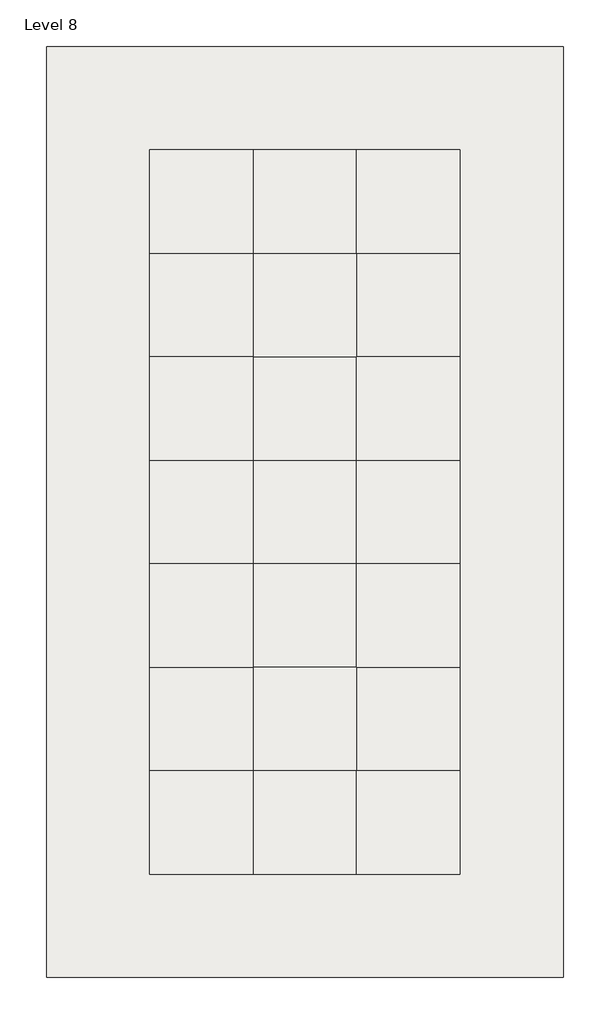
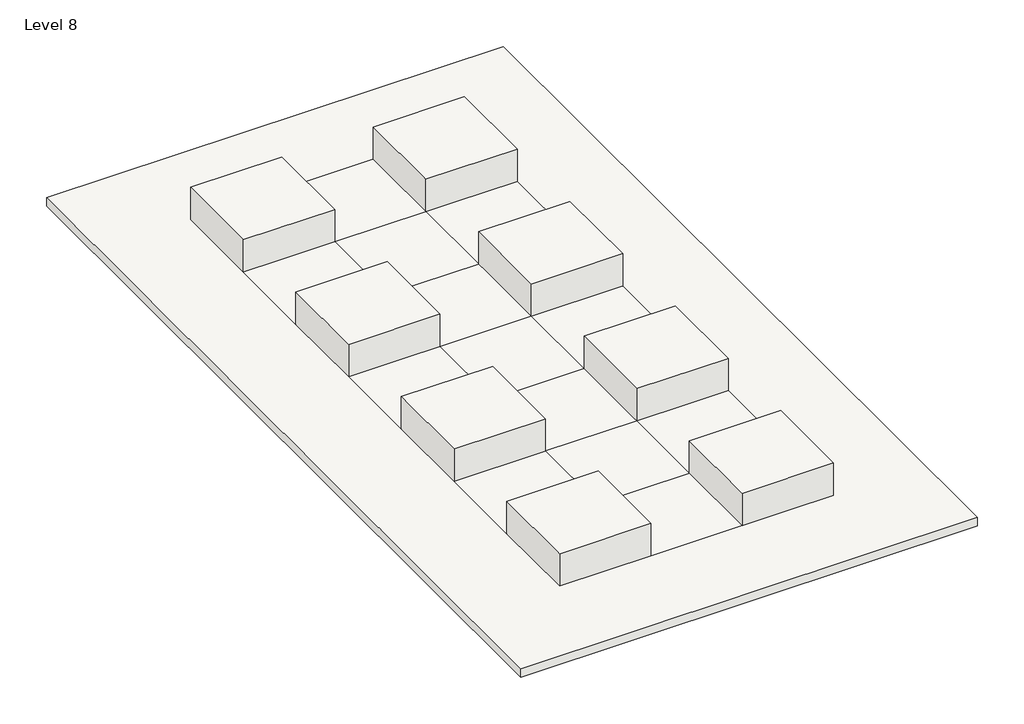
# One storey: 9 roofs.
"""IFC4 building model written with IfcOpenShell, lengths in millimetres."""

from ifc_helpers import new_model, si_unit, origin, place, context, project, spatial, faceted_brep, element, save

model = new_model("IFC4")

# Units and contexts
model_context = context("Model", 3, world=origin())
ifc_project = project(units=[si_unit("LENGTHUNIT", "METRE", prefix="MILLI")], contexts=[model_context])

# Site, building, storey
site = spatial("IfcSite", under=ifc_project)
building = spatial("IfcBuilding", under=site)
storey = spatial("IfcBuildingStorey", under=building, Name="Level 8", Elevation=32000.0)

# Roofs
placement = place(None, origin())
element("IfcRoof", 1, ObjectType="Bauder_RoofCoveringSystem_IntensiveGreenRoofSystem", at=placement, inside=storey, context=model_context, shape_type="Brep", body=[
    faceted_brep([(-674.7340554, 1676.2074539, 32000.0), (1325.2659446, 1676.2074539, 32000.0), (1325.2659446, -323.7925461, 32000.0), (-674.7340554, -323.7925461, 32000.0), (1325.2659446, 1676.2074539, 32949.8), (-674.7340554, 1676.2074539, 32949.8), (-674.7340554, -323.7925461, 32949.8), (1325.2659446, -323.7925461, 32949.8), (1325.2659446, 1676.2074539, 32200.0), (-674.7340554, 1676.2074539, 32200.0), (-674.7340554, -323.7925461, 32200.0), (1325.2659446, -323.7925461, 32200.0)], [[[0, 1, 2, 3]], [[4, 5, 6, 7]], [[5, 4, 8, 1, 0, 9]], [[6, 5, 9, 0, 3, 10]], [[7, 6, 10, 3, 2, 11]], [[4, 7, 11, 2, 1, 8]]]),
])
element("IfcRoof", 2, ObjectType="Bauder_RoofCoveringSystem_IntensiveGreenRoofSystem", at=placement, inside=storey, context=model_context, shape_type="Brep", body=[
    faceted_brep([(3325.2659446, 1676.2074539, 32000.0), (5325.2659446, 1676.2074539, 32000.0), (5325.2659446, -323.7925461, 32000.0), (3325.2659446, -323.7925461, 32000.0), (5325.2659446, 1676.2074539, 32949.8), (3325.2659446, 1676.2074539, 32949.8), (3325.2659446, -323.7925461, 32949.8), (5325.2659446, -323.7925461, 32949.8), (5325.2659446, 1676.2074539, 32200.0), (3325.2659446, 1676.2074539, 32200.0), (3325.2659446, -323.7925461, 32200.0), (5325.2659446, -323.7925461, 32200.0)], [[[0, 1, 2, 3]], [[4, 5, 6, 7]], [[5, 4, 8, 1, 0, 9]], [[6, 5, 9, 0, 3, 10]], [[7, 6, 10, 3, 2, 11]], [[4, 7, 11, 2, 1, 8]]]),
])
element("IfcRoof", 3, ObjectType="Bauder_RoofCoveringSystem_IntensiveGreenRoofSystem", at=placement, inside=storey, context=model_context, shape_type="Brep", body=[
    faceted_brep([(3325.2659446, -2323.7925461, 32000.0), (5325.2659446, -2323.7925461, 32000.0), (5325.2659446, -4323.7925461, 32000.0), (3325.2659446, -4323.7925461, 32000.0), (5325.2659446, -2323.7925461, 32949.8), (3325.2659446, -2323.7925461, 32949.8), (3325.2659446, -4323.7925461, 32949.8), (5325.2659446, -4323.7925461, 32949.8), (5325.2659446, -2323.7925461, 32200.0), (3325.2659446, -2323.7925461, 32200.0), (3325.2659446, -4323.7925461, 32200.0), (5325.2659446, -4323.7925461, 32200.0)], [[[0, 1, 2, 3]], [[4, 5, 6, 7]], [[5, 4, 8, 1, 0, 9]], [[6, 5, 9, 0, 3, 10]], [[7, 6, 10, 3, 2, 11]], [[4, 7, 11, 2, 1, 8]]]),
])
element("IfcRoof", 4, ObjectType="Bauder_RoofCoveringSystem_IntensiveGreenRoofSystem", at=placement, inside=storey, context=model_context, shape_type="Brep", body=[
    faceted_brep([(3325.2659446, -6323.7925461, 32000.0), (5325.2659446, -6323.7925461, 32000.0), (5325.2659446, -8323.7925461, 32000.0), (3325.2659446, -8323.7925461, 32000.0), (5325.2659446, -6323.7925461, 32949.8), (3325.2659446, -6323.7925461, 32949.8), (3325.2659446, -8323.7925461, 32949.8), (5325.2659446, -8323.7925461, 32949.8), (5325.2659446, -6323.7925461, 32200.0), (3325.2659446, -6323.7925461, 32200.0), (3325.2659446, -8323.7925461, 32200.0), (5325.2659446, -8323.7925461, 32200.0)], [[[0, 1, 2, 3]], [[4, 5, 6, 7]], [[5, 4, 8, 1, 0, 9]], [[6, 5, 9, 0, 3, 10]], [[7, 6, 10, 3, 2, 11]], [[4, 7, 11, 2, 1, 8]]]),
])
element("IfcRoof", 5, ObjectType="Bauder_RoofCoveringSystem_IntensiveGreenRoofSystem", at=placement, inside=storey, context=model_context, shape_type="Brep", body=[
    faceted_brep([(3325.2659446, -10323.7925461, 32000.0), (5325.2659446, -10323.7925461, 32000.0), (5325.2659446, -12323.7925461, 32000.0), (3325.2659446, -12323.7925461, 32000.0), (5325.2659446, -10323.7925461, 32949.8), (3325.2659446, -10323.7925461, 32949.8), (3325.2659446, -12323.7925461, 32949.8), (5325.2659446, -12323.7925461, 32949.8), (5325.2659446, -10323.7925461, 32200.0), (3325.2659446, -10323.7925461, 32200.0), (3325.2659446, -12323.7925461, 32200.0), (5325.2659446, -12323.7925461, 32200.0)], [[[0, 1, 2, 3]], [[4, 5, 6, 7]], [[5, 4, 8, 1, 0, 9]], [[6, 5, 9, 0, 3, 10]], [[7, 6, 10, 3, 2, 11]], [[4, 7, 11, 2, 1, 8]]]),
])
element("IfcRoof", 6, ObjectType="Bauder_RoofCoveringSystem_IntensiveGreenRoofSystem", at=placement, inside=storey, context=model_context, shape_type="Brep", body=[
    faceted_brep([(-674.7340554, -10323.7925461, 32000.0), (1325.2659446, -10323.7925461, 32000.0), (1325.2659446, -12323.7925461, 32000.0), (-674.7340554, -12323.7925461, 32000.0), (1325.2659446, -10323.7925461, 32949.8), (-674.7340554, -10323.7925461, 32949.8), (-674.7340554, -12323.7925461, 32949.8), (1325.2659446, -12323.7925461, 32949.8), (1325.2659446, -10323.7925461, 32200.0), (-674.7340554, -10323.7925461, 32200.0), (-674.7340554, -12323.7925461, 32200.0), (1325.2659446, -12323.7925461, 32200.0)], [[[0, 1, 2, 3]], [[4, 5, 6, 7]], [[5, 4, 8, 1, 0, 9]], [[6, 5, 9, 0, 3, 10]], [[7, 6, 10, 3, 2, 11]], [[4, 7, 11, 2, 1, 8]]]),
])
element("IfcRoof", 7, ObjectType="Bauder_RoofCoveringSystem_IntensiveGreenRoofSystem", at=placement, inside=storey, context=model_context, shape_type="Brep", body=[
    faceted_brep([(-674.7340554, -6323.7925461, 32000.0), (1325.2659446, -6323.7925461, 32000.0), (1325.2659446, -8323.7925461, 32000.0), (-674.7340554, -8323.7925461, 32000.0), (1325.2659446, -6323.7925461, 32949.8), (-674.7340554, -6323.7925461, 32949.8), (-674.7340554, -8323.7925461, 32949.8), (1325.2659446, -8323.7925461, 32949.8), (1325.2659446, -6323.7925461, 32200.0), (-674.7340554, -6323.7925461, 32200.0), (-674.7340554, -8323.7925461, 32200.0), (1325.2659446, -8323.7925461, 32200.0)], [[[0, 1, 2, 3]], [[4, 5, 6, 7]], [[5, 4, 8, 1, 0, 9]], [[6, 5, 9, 0, 3, 10]], [[7, 6, 10, 3, 2, 11]], [[4, 7, 11, 2, 1, 8]]]),
])
element("IfcRoof", 8, ObjectType="Bauder_RoofCoveringSystem_IntensiveGreenRoofSystem", at=placement, inside=storey, context=model_context, shape_type="Brep", body=[
    faceted_brep([(-674.7340554, -2323.7925461, 32000.0), (1325.2659446, -2323.7925461, 32000.0), (1325.2659446, -4323.7925461, 32000.0), (-674.7340554, -4323.7925461, 32000.0), (1325.2659446, -2323.7925461, 32949.8), (-674.7340554, -2323.7925461, 32949.8), (-674.7340554, -4323.7925461, 32949.8), (1325.2659446, -4323.7925461, 32949.8), (1325.2659446, -2323.7925461, 32200.0), (-674.7340554, -2323.7925461, 32200.0), (-674.7340554, -4323.7925461, 32200.0), (1325.2659446, -4323.7925461, 32200.0)], [[[0, 1, 2, 3]], [[4, 5, 6, 7]], [[5, 4, 8, 1, 0, 9]], [[6, 5, 9, 0, 3, 10]], [[7, 6, 10, 3, 2, 11]], [[4, 7, 11, 2, 1, 8]]]),
])
element("IfcRoof", 9, ObjectType="Roof_Concrete-200mm", at=placement, inside=storey, context=model_context, shape_type="Brep", body=[
    faceted_brep([(-2674.7340554, -14323.7925461, 32200.0), (-2674.7340554, -14323.7925461, 32000.0), (7325.2659446, -14323.7925461, 32000.0), (7325.2659446, -14323.7925461, 32200.0), (-2674.7340554, 3676.2074539, 32200.0), (-2674.7340554, 3676.2074539, 32000.0), (7325.2659446, 3676.2074539, 32200.0), (7325.2659446, 3676.2074539, 32000.0), (3325.2659446, 1676.2074539, 32200.0), (1325.2659446, 1676.2074539, 32200.0), (1325.2659446, -323.7925461, 32200.0), (3325.2659446, -323.7925461, 32200.0), (1325.2659446, 1676.2074539, 32000.0), (3325.2659446, 1676.2074539, 32000.0), (3325.2659446, -323.7925461, 32000.0), (1325.2659446, -323.7925461, 32000.0), (1325.2659446, -2323.7925461, 32200.0), (-674.7340554, -323.7925461, 32200.0), (-674.7340554, -2323.7925461, 32200.0), (3325.2659446, -2323.7925461, 32200.0), (5325.2659446, -2323.7925461, 32200.0), (5325.2659446, -323.7925461, 32200.0), (-674.7340554, -2323.7925461, 32000.0), (-674.7340554, -323.7925461, 32000.0), (1325.2659446, -2323.7925461, 32000.0), (3325.2659446, -2323.7925461, 32000.0), (5325.2659446, -323.7925461, 32000.0), (5325.2659446, -2323.7925461, 32000.0), (1325.2659446, -4323.7925461, 32200.0), (3325.2659446, -4323.7925461, 32200.0), (3325.2659446, -4323.7925461, 32000.0), (1325.2659446, -4323.7925461, 32000.0), (1325.2659446, -6323.7925461, 32200.0), (-674.7340554, -4323.7925461, 32200.0), (-674.7340554, -6323.7925461, 32200.0), (5325.2659446, -6323.7925461, 32200.0), (5325.2659446, -4323.7925461, 32200.0), (3325.2659446, -6323.7925461, 32200.0), (-674.7340554, -6323.7925461, 32000.0), (-674.7340554, -4323.7925461, 32000.0), (1325.2659446, -6323.7925461, 32000.0), (3325.2659446, -6323.7925461, 32000.0), (5325.2659446, -4323.7925461, 32000.0), (5325.2659446, -6323.7925461, 32000.0), (1325.2659446, -12323.7925461, 32200.0), (3325.2659446, -12323.7925461, 32200.0), (3325.2659446, -10323.7925461, 32200.0), (1325.2659446, -10323.7925461, 32200.0), (3325.2659446, -12323.7925461, 32000.0), (1325.2659446, -12323.7925461, 32000.0), (1325.2659446, -10323.7925461, 32000.0), (3325.2659446, -10323.7925461, 32000.0), (1325.2659446, -8323.7925461, 32200.0), (-674.7340554, -8323.7925461, 32200.0), (-674.7340554, -10323.7925461, 32200.0), (3325.2659446, -8323.7925461, 32200.0), (5325.2659446, -10323.7925461, 32200.0), (5325.2659446, -8323.7925461, 32200.0), (-674.7340554, -10323.7925461, 32000.0), (-674.7340554, -8323.7925461, 32000.0), (1325.2659446, -8323.7925461, 32000.0), (3325.2659446, -8323.7925461, 32000.0), (5325.2659446, -8323.7925461, 32000.0), (5325.2659446, -10323.7925461, 32000.0), (-674.7340554, 1676.2074539, 32000.0), (-674.7340554, 1676.2074539, 32200.0), (5325.2659446, 1676.2074539, 32200.0), (5325.2659446, 1676.2074539, 32000.0), (5325.2659446, -12323.7925461, 32000.0), (5325.2659446, -12323.7925461, 32200.0), (-674.7340554, -12323.7925461, 32000.0), (-674.7340554, -12323.7925461, 32200.0)], [[[0, 1, 2, 3]], [[1, 0, 4, 5]], [[6, 7, 5, 4]], [[3, 2, 7, 6]], [[8, 9, 10, 11]], [[12, 13, 14, 15]], [[16, 10, 17, 18]], [[11, 10, 16, 19]], [[20, 21, 11, 19]], [[22, 23, 15, 24]], [[15, 14, 25, 24]], [[25, 14, 26, 27]], [[19, 16, 28, 29]], [[24, 25, 30, 31]], [[32, 28, 33, 34]], [[35, 36, 29, 37]], [[38, 39, 31, 40]], [[41, 30, 42, 43]], [[44, 45, 46, 47]], [[48, 49, 50, 51]], [[47, 52, 53, 54]], [[47, 46, 55, 52]], [[56, 57, 55, 46]], [[58, 59, 60, 50]], [[51, 50, 60, 61]], [[51, 61, 62, 63]], [[52, 55, 37, 32]], [[29, 28, 32, 37]], [[61, 60, 40, 41]], [[31, 30, 41, 40]], [[9, 12, 15, 10]], [[10, 15, 23, 17]], [[17, 23, 64, 65]], [[12, 9, 65, 64]], [[66, 67, 26, 21]], [[21, 26, 14, 11]], [[11, 14, 13, 8]], [[67, 66, 8, 13]], [[20, 27, 42, 36]], [[36, 42, 30, 29]], [[29, 30, 25, 19]], [[27, 20, 19, 25]], [[16, 24, 31, 28]], [[28, 31, 39, 33]], [[33, 39, 22, 18]], [[24, 16, 18, 22]], [[32, 40, 60, 52]], [[52, 60, 59, 53]], [[53, 59, 38, 34]], [[40, 32, 34, 38]], [[35, 43, 62, 57]], [[57, 62, 61, 55]], [[55, 61, 41, 37]], [[43, 35, 37, 41]], [[56, 63, 68, 69]], [[69, 68, 48, 45]], [[45, 48, 51, 46]], [[63, 56, 46, 51]], [[47, 50, 49, 44]], [[44, 49, 70, 71]], [[71, 70, 58, 54]], [[50, 47, 54, 58]], [[4, 0, 3, 6], [9, 8, 66, 21, 20, 36, 35, 57, 56, 69, 45, 44, 71, 54, 53, 34, 33, 18, 17, 65]], [[7, 2, 1, 5], [13, 12, 64, 23, 22, 39, 38, 59, 58, 70, 49, 48, 68, 63, 62, 43, 42, 27, 26, 67]]]),
])

save(model, "model.ifc")

# Revit data of these elements
# Type "Bauder_RoofCoveringSystem_IntensiveGreenRoofSystem"
#   Keynote = "Q37"
#   Type IFC Predefined Type = "FLAT_ROOF"
#   Export Type to IFC As = "IfcRoofType"
#   Model = "Bauder Intensive Landscaping and Substrate - Intensive Green Roof System"
#   Manufacturer = "Bauder Ltd"
#   Type Comments = "Intensive Green Roof System"
#   URL = "http://www.bauder.co.uk/"
#   Description = "Bauder Intensive GreenRoof system incorporating Intensive Landscaping with Intensive Substrate, Filter Fleece, Mineral Drain, DSE60 Polyethylene Drainage and Protection Layer, FSM 1100 protection mat and PE Foil Polyethylene Separation-Slip Layer"
#   Assembly Code = "B3010"
#   NBSDescription = "Intensive green roof system"
#   NBSReference = "45-40-47/110"
#   BIMObjectName = "Bauder_RoofCoveringSystem_IntensiveGreenRoofSystem"
#   AccessibilityPerformance = "n/a"
#   CodePerformance = "n/a"
#   Color = "n/a"
#   Constituents = "n/a"
#   DurationUnit = "Year"
#   ExpectedLife = "n/a"
#   Features = "This BIM Object must be supported by a project specific specification from Bauder, incorporating system build-up, detail design and performance calculations if a full Bauder system guarantee is required. Please contact your local Bauder Representative or technical@bauder.co.uk"
#   Finish = "n/a"
#   Grade = "n/a"
#   Material = "n/a"
#   ModelReference = "Bauder Intensive Landscaping and Substrate - Intensive Green Roof System"
#   Name = "RoofCoveringSystem_Bauder_IntensiveGreenRoofSystem"
#   ReplacementCost = "n/a"
#   Shape = "n/a"
#   Size = "n/a"
#   SustainabilityPerformance = "Bauder Germany ISO14001: Certificate No.: 70499/03-15 e, Bauder UK ISO14001:Certificate No. 19ACM6595R, EN1271, BREEAM Credits Available"
#   WarrantyDescription = "Guarantee options could include ‘Product’, ‘Product and Workmanship’ and ‘Product, Workmanship and Design’ Guarantees. All guarantees available for this system are subject to the works being carried out in accordance with the Bauder specification and being installed by a Bauder Approved installer. For full details and further information regarding guarantees and alternative systems please contact your local Bauder Representative or technical@bauder.co.uk"
#   WarrantyDurationLabor = "n/a"
#   WarrantyDurationParts = "n/a\r\nn/a"
#   WarrantyDurationUnit = "Year"
#   WarrantyGuarantorLabor = "n/a"
#   WarrantyGuarantorParts = "technical@bauder.co.uk"
#   Certification = "n/a"
#   EdgeRestraints = "Perforated edge trim where required, refer to Bauder Project Specific Specification"
#   MoistureControlDrainageAncillaries = "n/a"
#   MoistureControlDrainageLayer = "Bauder DSE60 60 mm Polyethylene Drainage and Protection Layer with Bauder Mineral Drain Single size stone aggregate infill"
#   MoistureControlFilterMembrane = "Bauder Filter Fleece 1 mm Polypropylene Filter Fleece"
#   MoistureControlMoistureRetentionMat = "n/a"
#   PlantingSystemsAntierosionMat = "Jute Net where exposed, refer to Bauder Project Specific Specification"
#   PlantingSystemsPlantingMedium = "Bauder Intensive Substrate Recycled crushed brick, expanded clay shale and composted pine bark"
#   PlantingSystemsVegetation = "Bauder Intensive Landscaping"
#   PlantingSystemsVegetationBarrier = "20-40 mm Rounded-Washed Stones, refer to Bauder Project Specific Specification"
#   ProjectSpecificationAndDesign = "This BIM Object must be supported by a project specific specification from Bauder, incorporating system build-up, detail design and performance calculations if a full Bauder system warranty is required. Please contact your local Bauder Representative or technical@bauder.co.uk"
#   ProtectionProtectionLayer = "BauderGREEN FSM 1100 Protection Mat"
#   ProtectionRootBarrier = "As per project specific Bauder Specification"
#   ProtectionSeparationLayer = "2 layers of Bauder PE Foil 0.2 mm Polyethylene Separation-Slip Layer"
#   SystemManufacturer = "Bauder Ltd"
#   WarrantyConsiderations = "All guarantees available for this system are subject to the works being carried out in accordance with the Bauder specification and being installed by a Bauder Approved installer. For full details and further information regarding guarantees and alternative systems please contact your local Bauder Representative or technical@bauder.co.uk"
#   Update = "1900-12-31T23:59:59"
#   Documentation = "https://www.bauder.co.uk/technical-centre/technical-literature/system-brochures"
#   DocumentReference = "http://www.bauder.co.uk/"
#   IfcExportAs = "IfcRoofType"
#   IfcExportType = "FLAT_ROOF"
#   MethodOfMesurement = "n/a"
#   Process = "Replacement at service life intervals"
#   FireRating = "n/a"
#   _Author = "AM"
#   _AuthorizedBy = "bimstore"
#   _CreatedBy = "technical@bauder.co.uk"
#   _DistributedBy = "www.bimstore.co"
#   AssetType = "Fixed"
#   ClassificationName = "Uniclass2015"
#   ClassificationValue = "Ss_45_40_47_40"
#   CreatedBy = "technical@bauder.co.uk"
#   CreatedOn = "2023-02-10 T00:00:00"
#   DocumentationCertificates = "n/a"
#   DocumentationInstallationGuide = "https://www.bauder.co.uk/technical-centre"
#   DocumentationLiterature = "https://www.bauder.co.uk/technical-centre"
#   DocumentationMaintenance = "https://www.bauder.co.uk/technical-centre/maintenance-advice"
#   DocumentationTechnical = "https://www.bauder.co.uk/green-roofs/intensive-green-roofs"
#   ManufacturerName = "Bauder Ltd"
#   ModelNumber = "0910_INT-InS-FF-D6-F11-PE"
#   ProductionYear = "2023"
#   ReferencedStandard = "n/a"
#   SpareParts = "n/a"
#   TypeName = "Intensive Green Roof System"
#   NBSNote = "n/a"
#   NBSObjectName = "Bauder - Intensive green roof system"
#   NBSOfficeMasterTag = "n/a"
#   Ballast = "n/a"
#   CarrierMembraneFixing = "n/a"
#   CarrierMembraneType = "n/a"
#   FillToPerimeterUpstands = "n/a"
#   FilterLayer = "n/a"
#   InsulationFixing = "n/a"
#   InsulationType = "n/a"
#   LiquidAppliedWaterproofCoatingReinforcement = "n/a"
#   LiquidAppliedWaterproofCoatingSurfaceTreatment = "n/a"
#   LiquidAppliedWaterproofCoatingType = "n/a"
#   PreparationExistingSubstrates = "n/a"
#   PreparationHorizontalWork = "n/a"
#   PreparationSkirtingsAndVerticalWork = "n/a"
#   ProtectionLayer = "n/a"
#   SystemAccessories = "n/a"
#   WaterproofCoveringFirstLayerAttachment = "n/a"
#   WaterproofCoveringFirstLayerType = "n/a"
#   WaterproofCoveringIntermediateLayerAttachment = "n/a"
#   WaterproofCoveringIntermediateLayerType = "n/a"
#   WaterproofCoveringTopLayerAttachment = "n/a"
#   InsulationAttachment = "n/a"
#   IsolatingLayer = "n/a"
#   CarrierMembraneAttachment = "n/a"
#   LiquidAppliedWaterproofCoatingWearingCourse = "n/a"
#   VapourControlLayer = "n/a"
#   VapourControlLayerAttachment_Bauder = "n/a"
#   WaterproofCoveringJoints = "n/a"
#   WaterproofCoveringType = "n/a"
#   SeparatingLayer = "n/a"
#   WaterproofCoveringAccessories = "Yes"
#   WaterproofCoveringAttachment = "n/a"
#   UpperProtectionLayer = "n/a"
#   LowerProtectionLayer = "n/a"
#   WaterproofCoveringTopLayerType = "n/a"
#   DetailWorkAncillaryItems = "Detail as per project specific Bauder Specification"
#   DetailWorkCoverStrips = "Detail as per project specific Bauder Specification"
#   DetailWorkFlashings = "Detail as per project specific Bauder Specification"
#   DetailWorkSkirtingsAndUpstands = "Detail as per project specific Bauder Specification"
#   DetailWorkWeltedDrips = "Detail as per project specific Bauder Specification"
#   OverlayFixing = "n/a"
#   OverlayType = "n/a"
#   SurfaceProtection = "n/a"
#   VapourControlLayerAttachment = "n/a"
#   VapourControlLayerType = "n/a"
#   Cost = 0
#   NominalHeight = 0 mm
#   NominalLength = 0 mm
#   TotalArea = 0 m²
#   NominalDepth = 0 mm
#   IsExternal = yes
#   _BimSpecGuid = 0
#   _BSBibleVersion = 16
#   _CurrentRevision = 4
#   Layers, outside or top first: 300 mm "Bauder_Landscaping_Intensive" (function 5); 400 mm "Bauder_IntensiveSubstrate_BauderGREEN-SUB-IM-UK" (function 2); 1 mm "Bauder_FilterFleece_BauderGREEN-FV-125-100" (function 2); 40 mm "Bauder_DrainageBoard_BauderGREEN-DSE-40" (function 3); 8 mm "Bauder_ProtectionMat_BauderGREEN-FSM1100" (function 3); 200 mm "Concrete" (function 1); 0.8 mm "Bauder_SeparationAndSlipLayer_BauderGREEN-PE-02" (function 3)
# Type "Roof_Concrete-200mm"
#   Layers, outside or top first: 200 mm "Concrete" (function 1)
# Elements 1, 2, 3, 4, 5, 6, 7, 8 (IfcRoof, "Bauder_RoofCoveringSystem_IntensiveGreenRoofSystem")
#   built-in parameter 1001705 = 108.103 (stored number, unit not read)
#   built-in parameter 1001710 = 33615
#   Phase Created = New Construction
#   Materials on its faces: "Bauder_SeparationAndSlipLayer_BauderGREEN-PE-02", "Bauder_Landscaping_Intensive"
# Element 9 (IfcRoof, "Roof_Concrete-200mm")
#   built-in parameter 1001710 = 33615
#   Phase Created = New Construction
#   Materials on its faces: "Concrete"
# Materials
#   "Bauder_Landscaping_Intensive": class "Unassigned", colour RGB 62 68 37, transparency 0, Mtrl_Author = "AM", Mtrl_AuthorizedBy = "bimstore", Mtrl_DistributedBy = "www.bimstore.co", Mtrl_AccessibilityPerformance = "n/a", Mtrl_AssetIdentifier = "Please record on commissioning", Mtrl_AssetType = "Fixed", Mtrl_BarCode = "Please record on commissioning", Mtrl_ClassificationName = "Uniclass2015", Mtrl_ClassificationValue = "n/a", Mtrl_CodePerformance = "n/a", Mtrl_Color = "n/a", Mtrl_Constituents = "n/a", Mtrl_CreatedBy = "technical@bauder.co.uk", Mtrl_CreatedOn = "2023-02-10 T00:00:00", Mtrl_DocumentationCertificates = "https://www.bimstore.co/products/intensive-green-roof-system/document/product-certificates", Mtrl_DocumentationInstallationGuide = "https://www.bimstore.co/products/intensive-green-roof-system/document/installation-guide", Mtrl_DocumentationLiterature = "https://www.bimstore.co/products/intensive-green-roof-system/document/product-literature", Mtrl_DocumentationMaintenance = "https://www.bimstore.co/products/intensive-green-roof-system/document/maintenance-information", Mtrl_DocumentationTechnical = "https://www.bimstore.co/products/intensive-green-roof-system/document/technical-data-sheet", Mtrl_DurationUnit = "Year", Mtrl_Features = "n/a", Mtrl_Finish = "n/a", Mtrl_Grade = "n/a", Mtrl_InstallationDate = "Please record on commissioning", Mtrl_ManufacturerName = "Bauder Ltd", Mtrl_Material = "n/a", Mtrl_ModelNumber = "Intensive", Mtrl_ModelReference = "Landscaping", Mtrl_ProductionYear = "2023", Mtrl_ReferencedStandard = "n/a", Mtrl_Shape = "n/a", Mtrl_Size = "n/a", Mtrl_SpareParts = "n/a", Mtrl_TypeName = "Intensive", Mtrl_WarrantyDescription = "n/a", Mtrl_WarrantyDurationUnit = "Year", Mtrl_WarrantyGuarantorLabor = "n/a", Mtrl_WarrantyGuarantorParts = "technical@bauder.co.uk", Mtrl_WarrantyStartDate = "Please record on commissioning", Mtrl_IfcExportAs = "IfcRoofType", Mtrl_IfcExportType = "FLAT_ROOF", Mtrl_BIMObjectName = "Bauder_Landscaping_Intensive", Mtrl_NBSDescription = "n/a", Mtrl_NBSNote = "n/a", Mtrl_NBSObjectName = "n/a", Mtrl_NBSOfficeMasterTag = "n/a", Mtrl_NBSReference = "Q37", Mtrl_Ballast = "n/a", Mtrl_CarrierMembraneAttachment = "n/a", Mtrl_CarrierMembraneFixing = "n/a", Mtrl_CarrierMembraneType = "n/a", Mtrl_Certification = "Comply with GRO Green Roof Code of Practice and FLL Standards", Mtrl_DetailWorkAncillaryItems = "Detail as per project specific Bauder Specification", Mtrl_DetailWorkCoverStrips = "Detail as per project specific Bauder Specification", Mtrl_DetailWorkFlashings = "Detail as per project specific Bauder Specification", Mtrl_DetailWorkSkirtingsAndUpstands = "Detail as per project specific Bauder Specification", Mtrl_DetailWorkWeltedDrips = "Detail as per project specific Bauder Specification", Mtrl_EdgeRestraints = "Detail as per project specific Bauder Specification", Mtrl_FillToPerimeterUpstands = "n/a", Mtrl_FilterLayer = "n/a", Mtrl_InsulationAttachment = "As per project specific Bauder Specification", Mtrl_InsulationFixing = "As per project specific Bauder Specification", Mtrl_InsulationType = "As per project specific Bauder Specification", Mtrl_IsolatingLayer = "n/a", Mtrl_LiquidAppliedWaterproofCoatingReinforcement = "n/a", Mtrl_LiquidAppliedWaterproofCoatingSurfaceTreatment = "As per project specific Bauder Specification", Mtrl_LiquidAppliedWaterproofCoatingType = "As per project specific Bauder Specification", Mtrl_LiquidAppliedWaterproofCoatingWearingCourse = "As per project specific Bauder Specification", Mtrl_LowerProtectionLayer = "n/a", Mtrl_MoistureControlDrainageAncillaries = "n/a", Mtrl_MoistureControlDrainageLayer = "n/a", Mtrl_MoistureControlFilterMembrane = "n/a", Mtrl_MoistureControlMoistureRetentionMat = "n/a", Mtrl_OverlayFixing = "n/a", Mtrl_OverlayType = "n/a", Mtrl_PlantingSystemsAntierosionMat = "n/a", Mtrl_PlantingSystemsPlantingMedium = "As per project specific Bauder Specification", Mtrl_PlantingSystemsVegetation = "As per project specific Bauder Specification", Mtrl_PlantingSystemsVegetationBarrier = "As per project specific Bauder Specification", Mtrl_PreparationExistingSubstrates = "n/a", Mtrl_PreparationHorizontalWork = "n/a", Mtrl_PreparationSkirtingsAndVerticalWork = "n/a", Mtrl_ProjectSpecificationAndDesign = "This BIM Object must be supported by a project specific specification from Bauder, incorporating system build-up, detail design and performance calculations if a full Bauder system warranty is required. Please contact your local Bauder Representative or technical@bauder.co.uk", Mtrl_ProtectionLayer = "n/a", Mtrl_ProtectionProtectionLayer = "n/a", Mtrl_ProtectionRootBarrier = "As per project specific Bauder Specification", Mtrl_ProtectionSeparationLayer = "n/a", Mtrl_SeparatingLayer = "n/a", Mtrl_SurfaceProtection = "n/a", Mtrl_SystemAccessories = "n/a", Mtrl_SystemManufacturer = "Bauder Ltd", Mtrl_Update = "1900-12-31 T23:59:59", Mtrl_UpperProtectionLayer = "n/a", Mtrl_VapourControlLayerAttachment = "As per project specific Bauder Specification", Mtrl_VapourControlLayerAttachment_Bauder = "As per project specific Bauder Specification", Mtrl_VapourControlLayerType = "As per project specific Bauder Specification", Mtrl_WarrantyConsiderations = "All guarantees available for this system are subject to the works being carried out in accordance with the Bauder specification and being installed by a Bauder Approved installer. For full details and further information regarding guarantees and alternative systems please contact your local Bauder Representative or technical@bauder.co.uk", Mtrl_WaterproofCoveringAccessories = "As per project specific Bauder Specification", Mtrl_WaterproofCoveringAttachment = "As per project specific Bauder Specification", Mtrl_WaterproofCoveringFirstLayerAttachment = "As per project specific Bauder Specification", Mtrl_WaterproofCoveringFirstLayerType = "As per project specific Bauder Specification", Mtrl_WaterproofCoveringIntermediateLayerAttachment = "As per project specific Bauder Specification", Mtrl_WaterproofCoveringIntermediateLayerType = "As per project specific Bauder Specification", Mtrl_WaterproofCoveringJoints = "As per project specific Bauder Specification", Mtrl_WaterproofCoveringTopLayerAttachment = "As per project specific Bauder Specification", Mtrl_WaterproofCoveringTopLayerType = "As per project specific Bauder Specification", Mtrl_WaterproofCoveringType = "As per project specific Bauder Specification", Cost = 0, Mtrl_ReplacementCost = 0, Mtrl_NominalDepth = 0 mm, Mtrl_NominalHeight = 0 mm, Mtrl_NominalLength = 0 mm, Mtrl_BimSpecGuid = 0, Mtrl_BSBibleVersion = 17, Mtrl_CurrentRevision = 2, Mtrl_ExpectedLife = 0, Mtrl_SerialNumber = 0, Mtrl_WarrantyDurationLabor = 0, Mtrl_WarrantyDurationParts = 0
#   "Bauder_IntensiveSubstrate_BauderGREEN-SUB-IM-UK": class "Unassigned", colour RGB 255 255 255, transparency 0, Mtrl_Author = "AM", Mtrl_AuthorizedBy = "bimstore", Mtrl_DistributedBy = "www.bimstore.co", Mtrl_AccessibilityPerformance = "n/a", Mtrl_AssetIdentifier = "Please record on commissioning", Mtrl_AssetType = "Fixed", Mtrl_BarCode = "Please record on commissioning", Mtrl_ClassificationName = "Uniclass2015", Mtrl_ClassificationValue = "n/a", Mtrl_CodePerformance = "n/a", Mtrl_Color = "n/a", Mtrl_Constituents = "n/a", Mtrl_CreatedBy = "technical@bauder.co.uk", Mtrl_CreatedOn = "2023-02-10 T00:00:00", Mtrl_DocumentationCertificates = "https://www.bimstore.co/products/intensive-green-roof-system/document/product-certificates", Mtrl_DocumentationInstallationGuide = "https://www.bimstore.co/products/intensive-green-roof-system/document/installation-guide", Mtrl_DocumentationLiterature = "https://www.bimstore.co/products/intensive-green-roof-system/document/product-literature", Mtrl_DocumentationMaintenance = "https://www.bimstore.co/products/intensive-green-roof-system/document/maintenance-information", Mtrl_DocumentationTechnical = "https://www.bimstore.co/products/intensive-green-roof-system/document/technical-data-sheet", Mtrl_DurationUnit = "Year", Mtrl_Features = "n/a", Mtrl_Finish = "n/a", Mtrl_Grade = "n/a", Mtrl_InstallationDate = "Please record on commissioning", Mtrl_ManufacturerName = "Bauder Ltd", Mtrl_Material = "Expanded Clay Aggregate", Mtrl_ModelNumber = "BauderGREEN-SUB-IM-UK", Mtrl_ModelReference = "Intensive Substrate", Mtrl_ProductionYear = "2023", Mtrl_ReferencedStandard = "n/a", Mtrl_Shape = "n/a", Mtrl_Size = "n/a", Mtrl_SpareParts = "n/a", Mtrl_TypeName = "BauderGREEN-SUB-IM-UK", Mtrl_WarrantyDescription = "As part of Bauder system guarantee, per specification", Mtrl_WarrantyDurationUnit = "Year", Mtrl_WarrantyGuarantorLabor = "n/a", Mtrl_WarrantyGuarantorParts = "technical@bauder.co.uk", Mtrl_WarrantyStartDate = "Please record on commissioning", Mtrl_IfcExportAs = "IfcRoofType", Mtrl_IfcExportType = "FLAT_ROOF", Mtrl_BIMObjectName = "Bauder_IntensiveSubstrate_BauderGREEN-SUB-IM-UK", Mtrl_NBSDescription = "n/a", Mtrl_NBSNote = "n/a", Mtrl_NBSObjectName = "n/a", Mtrl_NBSOfficeMasterTag = "n/a", Mtrl_NBSReference = "Q37", Mtrl_Ballast = "n/a", Mtrl_CarrierMembraneAttachment = "n/a", Mtrl_CarrierMembraneFixing = "n/a", Mtrl_CarrierMembraneType = "n/a", Mtrl_Certification = "Comply with GRO Green Roof Code of Practice and FLL Standards", Mtrl_DetailWorkAncillaryItems = "Detail as per project specific Bauder Specification", Mtrl_DetailWorkCoverStrips = "Detail as per project specific Bauder Specification", Mtrl_DetailWorkFlashings = "Detail as per project specific Bauder Specification", Mtrl_DetailWorkSkirtingsAndUpstands = "Detail as per project specific Bauder Specification", Mtrl_DetailWorkWeltedDrips = "Detail as per project specific Bauder Specification", Mtrl_EdgeRestraints = "Detail as per project specific Bauder Specification", Mtrl_FillToPerimeterUpstands = "n/a", Mtrl_FilterLayer = "n/a", Mtrl_InsulationAttachment = "As per project specific Bauder Specification", Mtrl_InsulationFixing = "As per project specific Bauder Specification", Mtrl_InsulationType = "As per project specific Bauder Specification", Mtrl_IsolatingLayer = "n/a", Mtrl_LiquidAppliedWaterproofCoatingReinforcement = "As per project specific Bauder Specification", Mtrl_LiquidAppliedWaterproofCoatingSurfaceTreatment = "As per project specific Bauder Specification", Mtrl_LiquidAppliedWaterproofCoatingType = "As per project specific Bauder Specification", Mtrl_LiquidAppliedWaterproofCoatingWearingCourse = "As per project specific Bauder Specification", Mtrl_LowerProtectionLayer = "n/a", Mtrl_MoistureControlDrainageAncillaries = "n/a", Mtrl_MoistureControlDrainageLayer = "n/a", Mtrl_MoistureControlFilterMembrane = "n/a", Mtrl_MoistureControlMoistureRetentionMat = "n/a", Mtrl_OverlayFixing = "n/a", Mtrl_OverlayType = "n/a", Mtrl_PlantingSystemsAntierosionMat = "n/a", Mtrl_PlantingSystemsPlantingMedium = "As per project specific Bauder Specification", Mtrl_PlantingSystemsVegetation = "As per project specific Bauder Specification", Mtrl_PlantingSystemsVegetationBarrier = "As per project specific Bauder Specification", Mtrl_PreparationExistingSubstrates = "n/a", Mtrl_PreparationHorizontalWork = "n/a", Mtrl_PreparationSkirtingsAndVerticalWork = "n/a", Mtrl_ProjectSpecificationAndDesign = "This BIM Object must be supported by a project specific specification from Bauder, incorporating system build-up, detail design and performance calculations if a full Bauder system warranty is required. Please contact your local Bauder Representative or technical@bauder.co.uk", Mtrl_ProtectionLayer = "n/a", Mtrl_ProtectionProtectionLayer = "n/a", Mtrl_ProtectionRootBarrier = "As per project specific Bauder Specification", Mtrl_ProtectionSeparationLayer = "n/a", Mtrl_SeparatingLayer = "n/a", Mtrl_SurfaceProtection = "n/a", Mtrl_SystemAccessories = "n/a", Mtrl_SystemManufacturer = "Bauder Ltd", Mtrl_Update = "1900-12-31 T23:59:59", Mtrl_UpperProtectionLayer = "n/a", Mtrl_VapourControlLayerAttachment = "As per project specific Bauder Specification", Mtrl_VapourControlLayerAttachment_Bauder = "As per project specific Bauder Specification", Mtrl_VapourControlLayerType = "As per project specific Bauder Specification", Mtrl_WarrantyConsiderations = "All guarantees available for this system are subject to the works being carried out in accordance with the Bauder specification and being installed by a Bauder Approved installer. For full details and further information regarding guarantees and alternative systems please contact your local Bauder Representative or technical@bauder.co.uk", Mtrl_WaterproofCoveringAccessories = "As per project specific Bauder Specification", Mtrl_WaterproofCoveringAttachment = "As per project specific Bauder Specification", Mtrl_WaterproofCoveringFirstLayerAttachment = "As per project specific Bauder Specification", Mtrl_WaterproofCoveringFirstLayerType = "As per project specific Bauder Specification", Mtrl_WaterproofCoveringIntermediateLayerAttachment = "As per project specific Bauder Specification", Mtrl_WaterproofCoveringIntermediateLayerType = "As per project specific Bauder Specification", Mtrl_WaterproofCoveringJoints = "As per project specific Bauder Specification", Mtrl_WaterproofCoveringTopLayerAttachment = "As per project specific Bauder Specification", Mtrl_WaterproofCoveringTopLayerType = "As per project specific Bauder Specification", Mtrl_WaterproofCoveringType = "As per project specific Bauder Specification", Cost = 0, Mtrl_ReplacementCost = 0, Mtrl_NominalDepth = 200 mm, Mtrl_NominalHeight = 0 mm, Mtrl_NominalLength = 0 mm, Mtrl_BimSpecGuid = 0, Mtrl_BSBibleVersion = 17, Mtrl_CurrentRevision = 2, Mtrl_ExpectedLife = 0, Mtrl_SerialNumber = 0, Mtrl_WarrantyDurationLabor = 0, Mtrl_WarrantyDurationParts = 0
#   "Bauder_FilterFleece_BauderGREEN-FV-125-100": class "Unassigned", colour RGB 255 255 255, transparency 0, Mtrl_Author = "AM", Mtrl_AuthorizedBy = "bimstore", Mtrl_DistributedBy = "www.bimstore.co", Mtrl_AccessibilityPerformance = "n/a", Mtrl_AssetIdentifier = "Please record on commissioning", Mtrl_AssetType = "Fixed", Mtrl_BarCode = "Please record on commissioning", Mtrl_ClassificationName = "Uniclass2015", Mtrl_ClassificationValue = "n/a", Mtrl_CodePerformance = "n/a", Mtrl_Color = "n/a", Mtrl_Constituents = "n/a", Mtrl_CreatedBy = "technical@bauder.co.uk", Mtrl_CreatedOn = "2023-02-10 T00:00:00", Mtrl_DocumentationCertificates = "https://www.bimstore.co/products/extensive-green-roof-system-wildflower-blanket/document/product-certificates", Mtrl_DocumentationInstallationGuide = "https://www.bimstore.co/products/extensive-green-roof-system-wildflower-blanket/document/installation-guide", Mtrl_DocumentationLiterature = "https://www.bimstore.co/products/intensive-green-roof-system/document/product-literature", Mtrl_DocumentationMaintenance = "https://www.bimstore.co/products/extensive-green-roof-system-wildflower-blanket/document/maintenance-information", Mtrl_DocumentationTechnical = "https://www.bimstore.co/products/extensive-green-roof-system-wildflower-blanket/document/technical-data-sheet", Mtrl_DurationUnit = "Year", Mtrl_Features = "n/a", Mtrl_Finish = "n/a", Mtrl_Grade = "n/a", Mtrl_InstallationDate = "Please record on commissioning", Mtrl_ManufacturerName = "Bauder Ltd", Mtrl_Material = "Polypropylene Fleece", Mtrl_ModelNumber = "BauderGREEN-FV-125-100", Mtrl_ModelReference = "Filter Fleece", Mtrl_ProductionYear = "2023", Mtrl_ReferencedStandard = "n/a", Mtrl_Shape = "n/a", Mtrl_Size = "n/a", Mtrl_SpareParts = "n/a", Mtrl_TypeName = "BauderGREEN-FV-125-100", Mtrl_WarrantyDescription = "As part of Bauder system guarantee, per specification", Mtrl_WarrantyDurationUnit = "Year", Mtrl_WarrantyGuarantorLabor = "technical@bauder.co.uk", Mtrl_WarrantyGuarantorParts = "technical@bauder.co.uk", Mtrl_WarrantyStartDate = "Please record on commissioning", Mtrl_IfcExportAs = "IfcRoofType", Mtrl_IfcExportType = "FLAT_ROOF", Mtrl_BIMObjectName = "Bauder_FilterFleece_BauderGREEN-FV-125-100", Mtrl_NBSDescription = "n/a", Mtrl_NBSNote = "n/a", Mtrl_NBSObjectName = "n/a", Mtrl_NBSOfficeMasterTag = "n/a", Mtrl_NBSReference = "Q37", Mtrl_Ballast = "n/a", Mtrl_CarrierMembraneAttachment = "n/a", Mtrl_CarrierMembraneFixing = "n/a", Mtrl_CarrierMembraneType = "n/a", Mtrl_Certification = "Comply with GRO Green Roof Code of Practice and FLL Standards", Mtrl_DetailWorkAncillaryItems = "Detail as per project specific Bauder Specification", Mtrl_DetailWorkCoverStrips = "Detail as per project specific Bauder Specification", Mtrl_DetailWorkFlashings = "Detail as per project specific Bauder Specification", Mtrl_DetailWorkSkirtingsAndUpstands = "Detail as per project specific Bauder Specification", Mtrl_DetailWorkWeltedDrips = "Detail as per project specific Bauder Specification", Mtrl_EdgeRestraints = "Detail as per project specific Bauder Specification", Mtrl_FillToPerimeterUpstands = "n/a", Mtrl_FilterLayer = "n/a", Mtrl_InsulationAttachment = "As per project specific Bauder Specification", Mtrl_InsulationFixing = "As per project specific Bauder Specification", Mtrl_InsulationType = "As per project specific Bauder Specification", Mtrl_IsolatingLayer = "n/a", Mtrl_LiquidAppliedWaterproofCoatingReinforcement = "As per project specific Bauder Specification", Mtrl_LiquidAppliedWaterproofCoatingSurfaceTreatment = "As per project specific Bauder Specification", Mtrl_LiquidAppliedWaterproofCoatingType = "As per project specific Bauder Specification", Mtrl_LiquidAppliedWaterproofCoatingWearingCourse = "As per project specific Bauder Specification", Mtrl_LowerProtectionLayer = "n/a", Mtrl_MoistureControlDrainageAncillaries = "n/a", Mtrl_MoistureControlDrainageLayer = "n/a", Mtrl_MoistureControlFilterMembrane = "n/a", Mtrl_MoistureControlMoistureRetentionMat = "n/a", Mtrl_OverlayFixing = "n/a", Mtrl_OverlayType = "n/a", Mtrl_PlantingSystemsAntierosionMat = "n/a", Mtrl_PlantingSystemsPlantingMedium = "As per project specific Bauder Specification", Mtrl_PlantingSystemsVegetation = "As per project specific Bauder Specification", Mtrl_PlantingSystemsVegetationBarrier = "As per project specific Bauder Specification", Mtrl_PreparationExistingSubstrates = "n/a", Mtrl_PreparationHorizontalWork = "n/a", Mtrl_PreparationSkirtingsAndVerticalWork = "n/a", Mtrl_ProjectSpecificationAndDesign = "This BIM Object must be supported by a project specific specification from Bauder, incorporating system build-up, detail design and performance calculations if a full Bauder system warranty is required. Please contact your local Bauder Representative or technical@bauder.co.uk", Mtrl_ProtectionLayer = "n/a", Mtrl_ProtectionProtectionLayer = "n/a", Mtrl_ProtectionRootBarrier = "As per project specific Bauder Specification", Mtrl_ProtectionSeparationLayer = "n/a", Mtrl_SeparatingLayer = "n/a", Mtrl_SurfaceProtection = "n/a", Mtrl_SystemAccessories = "n/a", Mtrl_SystemManufacturer = "Bauder Ltd", Mtrl_Update = "1900-12-31 T23:59:59", Mtrl_UpperProtectionLayer = "n/a", Mtrl_VapourControlLayerAttachment = "As per project specific Bauder Specification", Mtrl_VapourControlLayerAttachment_Bauder = "As per project specific Bauder Specification", Mtrl_VapourControlLayerType = "As per project specific Bauder Specification", Mtrl_WarrantyConsiderations = "All guarantees available for this system are subject to the works being carried out in accordance with the Bauder specification and being installed by a Bauder Approved installer. For full details and further information regarding guarantees and alternative systems please contact your local Bauder Representative or technical@bauder.co.uk", Mtrl_WaterproofCoveringAccessories = "As per project specific Bauder Specification", Mtrl_WaterproofCoveringAttachment = "As per project specific Bauder Specification", Mtrl_WaterproofCoveringFirstLayerAttachment = "As per project specific Bauder Specification", Mtrl_WaterproofCoveringFirstLayerType = "As per project specific Bauder Specification", Mtrl_WaterproofCoveringIntermediateLayerAttachment = "As per project specific Bauder Specification", Mtrl_WaterproofCoveringIntermediateLayerType = "As per project specific Bauder Specification", Mtrl_WaterproofCoveringJoints = "As per project specific Bauder Specification", Mtrl_WaterproofCoveringTopLayerAttachment = "As per project specific Bauder Specification", Mtrl_WaterproofCoveringTopLayerType = "As per project specific Bauder Specification", Mtrl_WaterproofCoveringType = "As per project specific Bauder Specification", Cost = 0, Mtrl_ReplacementCost = 0, Mtrl_NominalDepth = 1 mm, Mtrl_NominalHeight = 0 mm, Mtrl_NominalLength = 0 mm, Mtrl_BimSpecGuid = 0, Mtrl_BSBibleVersion = 17, Mtrl_CurrentRevision = 2, Mtrl_ExpectedLife = 0, Mtrl_SerialNumber = 0, Mtrl_WarrantyDurationLabor = 0, Mtrl_WarrantyDurationParts = 0
#   "Bauder_DrainageBoard_BauderGREEN-DSE-40": class "Unassigned", colour RGB 255 255 255, transparency 0, Mtrl_Author = "AM", Mtrl_AuthorizedBy = "bimstore", Mtrl_DistributedBy = "www.bimstore.co", Mtrl_AccessibilityPerformance = "n/a", Mtrl_AssetIdentifier = "Please record on commissioning", Mtrl_AssetType = "Fixed", Mtrl_BarCode = "Please record on commissioning", Mtrl_ClassificationName = "Uniclass2015", Mtrl_ClassificationValue = "Pr_65_67_78_72", Mtrl_CodePerformance = "n/a", Mtrl_Color = "n/a", Mtrl_Constituents = "n/a", Mtrl_CreatedBy = "technical@bauder.co.uk", Mtrl_CreatedOn = "2023-02-10 T00:00:00", Mtrl_DocumentationCertificates = "https://www.bimstore.co/products/extensive-green-roof-system-wildflower-blanket/document/product-certificates", Mtrl_DocumentationInstallationGuide = "https://www.bimstore.co/products/extensive-green-roof-system-wildflower-blanket/document/installation-guide", Mtrl_DocumentationLiterature = "https://www.bimstore.co/products/extensive-green-roof-system-wildflower-blanket/document/product-literature", Mtrl_DocumentationMaintenance = "https://www.bimstore.co/products/extensive-green-roof-system-wildflower-blanket/document/maintenance-information", Mtrl_DocumentationTechnical = "https://www.bimstore.co/products/extensive-green-roof-system-wildflower-blanket/document/technical-data-sheet", Mtrl_DurationUnit = "Year", Mtrl_Features = "n/a", Mtrl_Finish = "n/a", Mtrl_Grade = "n/a", Mtrl_InstallationDate = "Please record on commissioning", Mtrl_ManufacturerName = "Bauder Ltd", Mtrl_Material = "Recycled High Density Polyethylene", Mtrl_ModelNumber = "BauderGREEN-DSE-40", Mtrl_ModelReference = "Drainage Board", Mtrl_ProductionYear = "2023", Mtrl_ReferencedStandard = "n/a", Mtrl_Shape = "n/a", Mtrl_Size = "n/a", Mtrl_SpareParts = "n/a", Mtrl_TypeName = "BauderGREEN-DSE-40", Mtrl_WarrantyDescription = "As part of Bauder system guarantee, per specification", Mtrl_WarrantyDurationUnit = "Year", Mtrl_WarrantyGuarantorLabor = "technical@bauder.co.uk", Mtrl_WarrantyGuarantorParts = "technical@bauder.co.uk", Mtrl_WarrantyStartDate = "Please record on commissioning", Mtrl_IfcExportAs = "IfcRoofType", Mtrl_IfcExportType = "FLAT_ROOF", Mtrl_BIMObjectName = "Bauder_DrainageBoard_BauderGREEN-DSE-40", Mtrl_NBSDescription = "n/a", Mtrl_NBSNote = "n/a", Mtrl_NBSObjectName = "n/a", Mtrl_NBSOfficeMasterTag = "n/a", Mtrl_NBSReference = "Q37", Mtrl_Ballast = "n/a", Mtrl_CarrierMembraneAttachment = "n/a", Mtrl_CarrierMembraneFixing = "n/a", Mtrl_CarrierMembraneType = "n/a", Mtrl_Certification = "Comply with GRO Green Roof Code of Practice and FLL Standards", Mtrl_DetailWorkAncillaryItems = "Detail as per project specific Bauder Specification", Mtrl_DetailWorkCoverStrips = "Detail as per project specific Bauder Specification", Mtrl_DetailWorkFlashings = "Detail as per project specific Bauder Specification", Mtrl_DetailWorkSkirtingsAndUpstands = "Detail as per project specific Bauder Specification", Mtrl_DetailWorkWeltedDrips = "Detail as per project specific Bauder Specification", Mtrl_EdgeRestraints = "Detail as per project specific Bauder Specification", Mtrl_FillToPerimeterUpstands = "n/a", Mtrl_FilterLayer = "n/a", Mtrl_InsulationAttachment = "As per project specific Bauder Specification", Mtrl_InsulationFixing = "As per project specific Bauder Specification", Mtrl_InsulationType = "As per project specific Bauder Specification", Mtrl_IsolatingLayer = "n/a", Mtrl_LiquidAppliedWaterproofCoatingReinforcement = "As per project specific Bauder Specification", Mtrl_LiquidAppliedWaterproofCoatingSurfaceTreatment = "As per project specific Bauder Specification", Mtrl_LiquidAppliedWaterproofCoatingType = "As per project specific Bauder Specification", Mtrl_LiquidAppliedWaterproofCoatingWearingCourse = "As per project specific Bauder Specification", Mtrl_LowerProtectionLayer = "n/a", Mtrl_MoistureControlDrainageAncillaries = "n/a", Mtrl_MoistureControlDrainageLayer = "n/a", Mtrl_MoistureControlFilterMembrane = "n/a", Mtrl_MoistureControlMoistureRetentionMat = "n/a", Mtrl_OverlayFixing = "n/a", Mtrl_OverlayType = "n/a", Mtrl_PlantingSystemsAntierosionMat = "n/a", Mtrl_PlantingSystemsPlantingMedium = "As per project specific Bauder Specification", Mtrl_PlantingSystemsVegetation = "As per project specific Bauder Specification", Mtrl_PlantingSystemsVegetationBarrier = "As per project specific Bauder Specification", Mtrl_PreparationExistingSubstrates = "n/a", Mtrl_PreparationHorizontalWork = "n/a", Mtrl_PreparationSkirtingsAndVerticalWork = "n/a", Mtrl_ProjectSpecificationAndDesign = "This BIM Object must be supported by a project specific specification from Bauder, incorporating system build-up, detail design and performance calculations if a full Bauder system warranty is required. Please contact your local Bauder Representative or technical@bauder.co.uk", Mtrl_ProtectionLayer = "n/a", Mtrl_ProtectionProtectionLayer = "n/a", Mtrl_ProtectionRootBarrier = "As per project specific Bauder Specification", Mtrl_ProtectionSeparationLayer = "n/a", Mtrl_SeparatingLayer = "n/a", Mtrl_SurfaceProtection = "n/a", Mtrl_SystemAccessories = "n/a", Mtrl_SystemManufacturer = "Bauder Ltd", Mtrl_Update = "1900-12-31 T23:59:59", Mtrl_UpperProtectionLayer = "n/a", Mtrl_VapourControlLayerAttachment = "As per project specific Bauder Specification", Mtrl_VapourControlLayerAttachment_Bauder = "As per project specific Bauder Specification", Mtrl_VapourControlLayerType = "As per project specific Bauder Specification", Mtrl_WarrantyConsiderations = "All guarantees available for this system are subject to the works being carried out in accordance with the Bauder specification and being installed by a Bauder Approved installer. For full details and further information regarding guarantees and alternative systems please contact your local Bauder Representative or technical@bauder.co.uk", Mtrl_WaterproofCoveringAccessories = "As per project specific Bauder Specification", Mtrl_WaterproofCoveringAttachment = "As per project specific Bauder Specification", Mtrl_WaterproofCoveringFirstLayerAttachment = "As per project specific Bauder Specification", Mtrl_WaterproofCoveringFirstLayerType = "As per project specific Bauder Specification", Mtrl_WaterproofCoveringIntermediateLayerAttachment = "As per project specific Bauder Specification", Mtrl_WaterproofCoveringIntermediateLayerType = "As per project specific Bauder Specification", Mtrl_WaterproofCoveringJoints = "As per project specific Bauder Specification", Mtrl_WaterproofCoveringTopLayerAttachment = "As per project specific Bauder Specification", Mtrl_WaterproofCoveringTopLayerType = "As per project specific Bauder Specification", Mtrl_WaterproofCoveringType = "As per project specific Bauder Specification", Cost = 0, Mtrl_ReplacementCost = 0, Mtrl_NominalDepth = 40 mm, Mtrl_NominalHeight = 0 mm, Mtrl_NominalLength = 0 mm, Mtrl_BimSpecGuid = 0, Mtrl_BSBibleVersion = 17, Mtrl_CurrentRevision = 2, Mtrl_ExpectedLife = 0, Mtrl_SerialNumber = 0, Mtrl_WarrantyDurationLabor = 0, Mtrl_WarrantyDurationParts = 0
#   "Bauder_ProtectionMat_BauderGREEN-FSM1100": class "Unassigned", colour RGB 255 255 255, transparency 0, Mtrl_Author = "AM", Mtrl_AuthorizedBy = "bimstore", Mtrl_DistributedBy = "www.bimstore.co", Mtrl_AccessibilityPerformance = "n/a", Mtrl_AssetIdentifier = "Please record on commissioning", Mtrl_AssetType = "Fixed", Mtrl_BarCode = "Please record on commissioning", Mtrl_ClassificationName = "Uniclass2015", Mtrl_ClassificationValue = "Pr_20_96_71_64", Mtrl_CodePerformance = "n/a", Mtrl_Color = "n/a", Mtrl_Constituents = "n/a", Mtrl_CreatedBy = "technical@bauder.co.uk", Mtrl_CreatedOn = "2023-05-02 T00:00:00", Mtrl_DocumentationCertificates = "https://www.bimstore.co/products/intensive-green-roof-system/document/product-certificates", Mtrl_DocumentationInstallationGuide = "https://www.bimstore.co/products/intensive-green-roof-system/document/installation-guide", Mtrl_DocumentationLiterature = "https://www.bimstore.co/products/intensive-green-roof-system/document/product-literature", Mtrl_DocumentationMaintenance = "https://www.bimstore.co/products/intensive-green-roof-system/document/maintenance-information", Mtrl_DocumentationTechnical = "https://www.bimstore.co/products/intensive-green-roof-system/document/technical-data-sheet", Mtrl_DurationUnit = "Year", Mtrl_Features = "n/a", Mtrl_Finish = "n/a", Mtrl_Grade = "n/a", Mtrl_InstallationDate = "Please record on commissioning", Mtrl_ManufacturerName = "Bauder Ltd", Mtrl_Material = "Polyester and Polypropylene Fibre", Mtrl_ModelNumber = "BauderGREEN FSM1100", Mtrl_ModelReference = "Protection Mat", Mtrl_ProductionYear = "2023", Mtrl_ReferencedStandard = "n/a", Mtrl_Shape = "n/a", Mtrl_Size = "n/a", Mtrl_SpareParts = "n/a", Mtrl_TypeName = "BauderGREEN FSM1100", Mtrl_WarrantyDescription = "As part of Bauder system guarantee, per specification", Mtrl_WarrantyDurationUnit = "Year", Mtrl_WarrantyGuarantorLabor = "n/a", Mtrl_WarrantyGuarantorParts = "technical@bauder.co.uk", Mtrl_WarrantyStartDate = "Please record on commissioning", Mtrl_IfcExportAs = "IfcRoofType", Mtrl_IfcExportType = "FLAT_ROOF", Mtrl_BIMObjectName = "Bauder_ProtectionMat_BauderGREEN-FSM1100", Mtrl_NBSDescription = "n/a", Mtrl_NBSNote = "n/a", Mtrl_NBSObjectName = "n/a", Mtrl_NBSOfficeMasterTag = "n/a", Mtrl_NBSReference = "Q37", Mtrl_Ballast = "n/a", Mtrl_CarrierMembraneAttachment = "n/a", Mtrl_CarrierMembraneFixing = "n/a", Mtrl_CarrierMembraneType = "n/a", Mtrl_Certification = "Comply with GRO Green Roof Code of Practice and FLL Standards", Mtrl_DetailWorkAncillaryItems = "Detail as per project specific Bauder Specification", Mtrl_DetailWorkCoverStrips = "Detail as per project specific Bauder Specification", Mtrl_DetailWorkFlashings = "Detail as per project specific Bauder Specification", Mtrl_DetailWorkSkirtingsAndUpstands = "Detail as per project specific Bauder Specification", Mtrl_DetailWorkWeltedDrips = "Detail as per project specific Bauder Specification", Mtrl_EdgeRestraints = "Detail as per project specific Bauder Specification", Mtrl_FillToPerimeterUpstands = "n/a", Mtrl_FilterLayer = "n/a", Mtrl_InsulationAttachment = "As per project specific Bauder Specification", Mtrl_InsulationFixing = "As per project specific Bauder Specification", Mtrl_InsulationType = "As per project specific Bauder Specification", Mtrl_IsolatingLayer = "n/a", Mtrl_LiquidAppliedWaterproofCoatingReinforcement = "As per project specific Bauder Specification", Mtrl_LiquidAppliedWaterproofCoatingSurfaceTreatment = "As per project specific Bauder Specification", Mtrl_LiquidAppliedWaterproofCoatingType = "As per project specific Bauder Specification", Mtrl_LiquidAppliedWaterproofCoatingWearingCourse = "As per project specific Bauder Specification", Mtrl_LowerProtectionLayer = "n/a", Mtrl_MoistureControlDrainageAncillaries = "n/a", Mtrl_MoistureControlDrainageLayer = "n/a", Mtrl_MoistureControlFilterMembrane = "n/a", Mtrl_MoistureControlMoistureRetentionMat = "n/a", Mtrl_OverlayFixing = "n/a", Mtrl_OverlayType = "n/a", Mtrl_PlantingSystemsAntierosionMat = "n/a", Mtrl_PlantingSystemsPlantingMedium = "As per project specific Bauder Specification", Mtrl_PlantingSystemsVegetation = "As per project specific Bauder Specification", Mtrl_PlantingSystemsVegetationBarrier = "As per project specific Bauder Specification", Mtrl_PreparationExistingSubstrates = "n/a", Mtrl_PreparationHorizontalWork = "n/a", Mtrl_PreparationSkirtingsAndVerticalWork = "n/a", Mtrl_ProjectSpecificationAndDesign = "This BIM Object must be supported by a project specific specification from Bauder, incorporating system build-up, detail design and performance calculations if a full Bauder system warranty is required. Please contact your local Bauder Representative or technical@bauder.co.uk", Mtrl_ProtectionLayer = "n/a", Mtrl_ProtectionProtectionLayer = "n/a", Mtrl_ProtectionRootBarrier = "As per project specific Bauder Specification", Mtrl_ProtectionSeparationLayer = "n/a", Mtrl_SeparatingLayer = "n/a", Mtrl_SurfaceProtection = "n/a", Mtrl_SystemAccessories = "n/a", Mtrl_SystemManufacturer = "Bauder Ltd", Mtrl_Update = "1900-12-31 T23:59:59", Mtrl_UpperProtectionLayer = "n/a", Mtrl_VapourControlLayerAttachment = "As per project specific Bauder Specification", Mtrl_VapourControlLayerAttachment_Bauder = "As per project specific Bauder Specification", Mtrl_VapourControlLayerType = "As per project specific Bauder Specification", Mtrl_WarrantyConsiderations = "All guarantees available for this system are subject to the works being carried out in accordance with the Bauder specification and being installed by a Bauder Approved installer. For full details and further information regarding guarantees and alternative systems please contact your local Bauder Representative or technical@bauder.co.uk", Mtrl_WaterproofCoveringAccessories = "As per project specific Bauder Specification", Mtrl_WaterproofCoveringAttachment = "As per project specific Bauder Specification", Mtrl_WaterproofCoveringFirstLayerAttachment = "As per project specific Bauder Specification", Mtrl_WaterproofCoveringFirstLayerType = "As per project specific Bauder Specification", Mtrl_WaterproofCoveringIntermediateLayerAttachment = "As per project specific Bauder Specification", Mtrl_WaterproofCoveringIntermediateLayerType = "As per project specific Bauder Specification", Mtrl_WaterproofCoveringJoints = "As per project specific Bauder Specification", Mtrl_WaterproofCoveringTopLayerAttachment = "As per project specific Bauder Specification", Mtrl_WaterproofCoveringTopLayerType = "As per project specific Bauder Specification", Mtrl_WaterproofCoveringType = "As per project specific Bauder Specification", Cost = 0, Mtrl_ReplacementCost = 0, Mtrl_NominalDepth = 8 mm, Mtrl_NominalHeight = 0 mm, Mtrl_NominalLength = 0 mm, Mtrl_BimSpecGuid = 0, Mtrl_BSBibleVersion = 17, Mtrl_CurrentRevision = 2, Mtrl_ExpectedLife = 0, Mtrl_SerialNumber = 0, Mtrl_WarrantyDurationLabor = 0, Mtrl_WarrantyDurationParts = 0
#   "Concrete": class "Concrete", colour RGB 120 120 120, transparency 0, Description = "Portland Cement Concrete", Cost = 0
